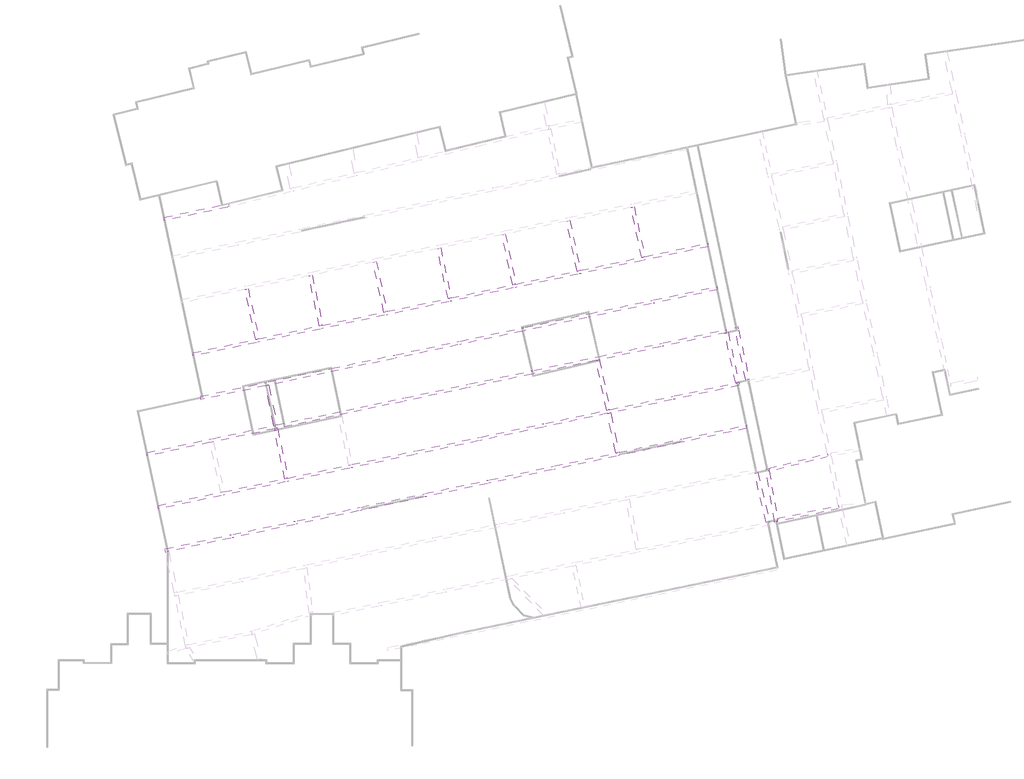
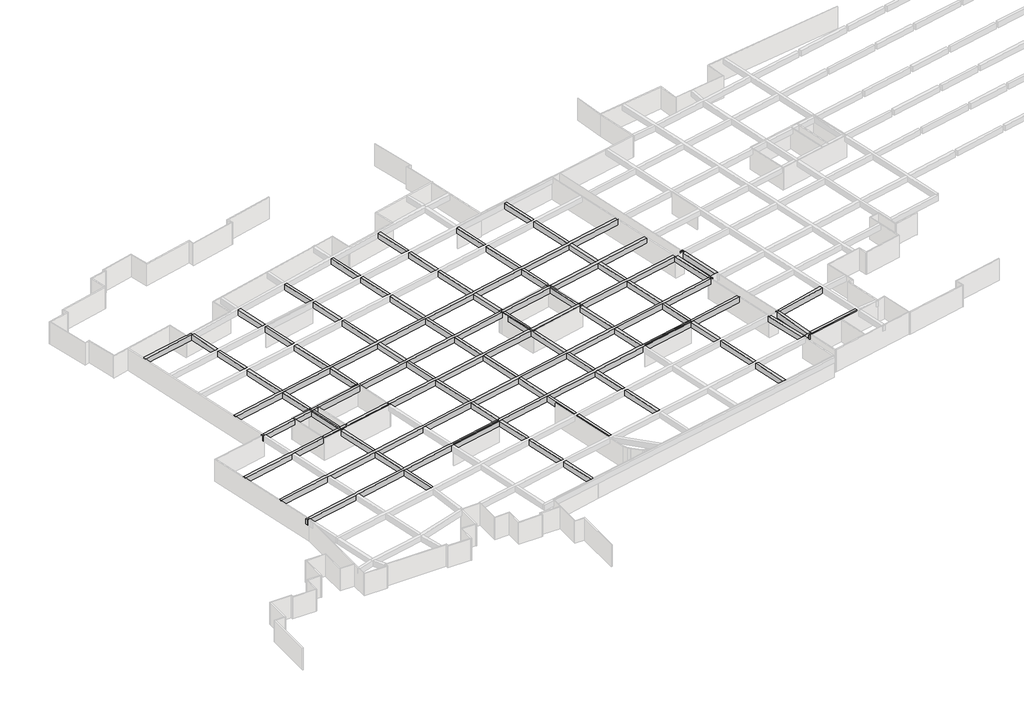
# One storey, part 8 of 14: 23 beams.
"""IFC4 building model written with IfcOpenShell, lengths in millimetres."""

from ifc_helpers import new_model, si_unit, frame, origin, place, context, project, spatial, polyline, outline, extrude, faceted_brep, element, save

model = new_model("IFC4")

# Units and contexts
model_context = context("Model", 3, world=origin())
ifc_project = project(units=[si_unit("LENGTHUNIT", "METRE", prefix="MILLI")], contexts=[model_context])

# Site, building, storey
site = spatial("IfcSite", under=ifc_project)
building = spatial("IfcBuilding", under=site)
storey = spatial("IfcBuildingStorey", under=building, Name="户型图", Elevation=0.0)

# Beams
placement = place(None, origin())
element("IfcBeam", 1, ObjectType="混凝土 - 矩形梁 : KL_beam", at=placement, inside=storey, context=model_context, shape_type="Brep", body=[
    faceted_brep([(-335089.4441213, -155154.5631684, 3300.0), (-335089.4441213, -155154.5631684, 2500.0), (-335006.2794449, -155545.8222087, 2500.0), (-335006.2794449, -155545.8222087, 3300.0), (-327178.3172304, -153881.9374755, 3300.0), (-327267.044724, -153491.8608485, 3300.0), (-327376.7281592, -153924.1110203, 3300.0), (-327178.3172304, -153881.9374755, 2500.0), (-327376.7281592, -153924.1110203, 2500.0), (-327267.044724, -153491.8608485, 2500.0)], [[[0, 1, 2, 3]], [[4, 5, 0, 3, 6]], [[7, 4, 6, 3, 2, 8]], [[9, 7, 8, 2, 1]], [[5, 9, 1, 0]], [[5, 4, 7, 9]]]),
])
element("IfcBeam", 2, ObjectType="混凝土 - 矩形梁 : KL_beam", at=placement, inside=storey, context=model_context, shape_type="Brep", body=[
    faceted_brep([(-269078.2925997, -158315.8590101, 3300.0), (-268995.1279234, -158707.1180504, 3300.0), (-268995.1279234, -158707.1180504, 2500.0), (-269078.2925997, -158315.8590101, 2500.0), (-331592.6839102, -171603.7030819, 3300.0), (-331592.6839102, -171603.7030819, 2500.0), (-331509.5192339, -171994.9621222, 2500.0), (-331509.5192339, -171994.9621222, 3300.0), (-276698.1734204, -159935.5146776, 3300.0), (-277089.4324607, -160018.679354, 3300.0), (-284525.3700507, -161599.2366809, 3300.0), (-284916.629091, -161682.4013572, 3300.0), (-292343.5420768, -163261.0404453, 3300.0), (-292734.8011171, -163344.2051217, 3300.0), (-300204.2486812, -164931.8852135, 3300.0), (-300595.5077215, -165015.0498898, 3300.0), (-308006.2318604, -166590.2479322, 3300.0), (-308397.4910792, -166673.4126465, 3300.0), (-315818.4231217, -168250.7804458, 3300.0), (-316209.682162, -168333.9451222, 3300.0), (-323572.2444184, -169898.9060405, 3300.0), (-323963.5034587, -169982.0707168, 3300.0), (-323880.3387823, -170373.3297571, 3300.0), (-323489.0797421, -170290.1650808, 3300.0), (-316126.5174857, -168725.2041625, 3300.0), (-315735.2584454, -168642.0394861, 3300.0), (-308313.9526955, -167064.5922528, 3300.0), (-307922.6934768, -166981.4275386, 3300.0), (-300512.3430452, -165406.3089301, 3300.0), (-300121.0840049, -165323.1442537, 3300.0), (-292651.6364408, -163735.4641619, 3300.0), (-292260.3774005, -163652.2994856, 3300.0), (-284833.4644147, -162073.6603975, 3300.0), (-284442.2053744, -161990.4957212, 3300.0), (-277006.2677843, -160409.9383943, 3300.0), (-276615.008744, -160326.7737179, 3300.0), (-323880.3387823, -170373.3297571, 2500.0), (-323489.0797421, -170290.1650808, 2500.0), (-316126.5174857, -168725.2041625, 2500.0), (-315735.2584454, -168642.0394861, 2500.0), (-308313.9526955, -167064.5922528, 2500.0), (-307922.6934768, -166981.4275386, 2500.0), (-300512.3430452, -165406.3089301, 2500.0), (-300121.0840049, -165323.1442537, 2500.0), (-292651.6364408, -163735.4641619, 2500.0), (-292260.3774005, -163652.2994856, 2500.0), (-284833.4644147, -162073.6603975, 2500.0), (-284442.2053744, -161990.4957212, 2500.0), (-277006.2677843, -160409.9383943, 2500.0), (-276615.008744, -160326.7737179, 2500.0), (-323963.5034587, -169982.0707168, 2500.0), (-323572.2444184, -169898.9060405, 2500.0), (-316209.682162, -168333.9451222, 2500.0), (-315818.4231217, -168250.7804458, 2500.0), (-308397.4910792, -166673.4126465, 2500.0), (-308006.2318604, -166590.2479322, 2500.0), (-300595.5077215, -165015.0498898, 2500.0), (-300204.2486812, -164931.8852135, 2500.0), (-292734.8011171, -163344.2051217, 2500.0), (-292343.5420768, -163261.0404453, 2500.0), (-284916.629091, -161682.4013572, 2500.0), (-284525.3700507, -161599.2366809, 2500.0), (-277089.4324607, -160018.679354, 2500.0), (-276698.1734204, -159935.5146776, 2500.0)], [[[0, 1, 2, 3]], [[4, 5, 6, 7]], [[1, 0, 8, 9, 10, 11, 12, 13, 14, 15, 16, 17, 18, 19, 20, 21, 4, 7, 22, 23, 24, 25, 26, 27, 28, 29, 30, 31, 32, 33, 34, 35]], [[2, 1, 35, 34, 33, 32, 31, 30, 29, 28, 27, 26, 25, 24, 23, 22, 7, 6, 36, 37, 38, 39, 40, 41, 42, 43, 44, 45, 46, 47, 48, 49]], [[3, 2, 49, 48, 47, 46, 45, 44, 43, 42, 41, 40, 39, 38, 37, 36, 6, 5, 50, 51, 52, 53, 54, 55, 56, 57, 58, 59, 60, 61, 62, 63]], [[0, 3, 63, 62, 61, 60, 59, 58, 57, 56, 55, 54, 53, 52, 51, 50, 5, 4, 21, 20, 19, 18, 17, 16, 15, 14, 13, 12, 11, 10, 9, 8]]]),
])
element("IfcBeam", 3, ObjectType="混凝土 - 矩形梁 : KL_beam", at=placement, inside=storey, context=model_context, shape_type="Brep", body=[
    faceted_brep([(-267962.3983208, -163565.7288339, 3300.0), (-267879.2336445, -163956.9878742, 3300.0), (-267879.2336445, -163956.9878742, 2500.0), (-267962.3983208, -163565.7288339, 2500.0), (-275582.2791414, -165185.3845014, 3300.0), (-275973.5381817, -165268.5491778, 3300.0), (-283409.4757718, -166849.1065047, 3300.0), (-283800.7348121, -166932.271181, 3300.0), (-291227.6477979, -168510.9102691, 3300.0), (-291618.9068381, -168594.0749454, 3300.0), (-299088.3544023, -170181.7550372, 3300.0), (-299479.6134426, -170264.9197136, 3300.0), (-306885.3232191, -171839.0519204, 3300.0), (-307276.5824379, -171922.2166347, 3300.0), (-314702.5288428, -173500.6502696, 3300.0), (-315093.787883, -173583.814946, 3300.0), (-322456.3501394, -175148.7758643, 3300.0), (-322847.6091797, -175231.9405406, 3300.0), (-330672.7899856, -176895.2340671, 3300.0), (-330589.6253093, -177286.4931074, 3300.0), (-330198.366269, -177203.3284311, 3300.0), (-322764.4445034, -175623.1995809, 3300.0), (-322373.1854631, -175540.0349045, 3300.0), (-307193.0440543, -172313.396241, 3300.0), (-306801.7848355, -172230.2315268, 3300.0), (-299396.4487662, -170656.1787539, 3300.0), (-299005.1897259, -170573.0140775, 3300.0), (-291535.7421618, -168985.3339857, 3300.0), (-291144.4831215, -168902.1693094, 3300.0), (-283717.5701358, -167323.5302213, 3300.0), (-283326.3110955, -167240.365545, 3300.0), (-275890.3735054, -165659.8082181, 3300.0), (-275499.1144651, -165576.6435417, 3300.0), (-330589.6253093, -177286.4931074, 2500.0), (-330198.366269, -177203.3284311, 2500.0), (-322764.4445034, -175623.1995809, 2500.0), (-322373.1854631, -175540.0349045, 2500.0), (-307193.0440543, -172313.396241, 2500.0), (-306801.7848355, -172230.2315268, 2500.0), (-299396.4487662, -170656.1787539, 2500.0), (-299005.1897259, -170573.0140775, 2500.0), (-291535.7421618, -168985.3339857, 2500.0), (-291144.4831215, -168902.1693094, 2500.0), (-283717.5701358, -167323.5302213, 2500.0), (-283326.3110955, -167240.365545, 2500.0), (-275890.3735054, -165659.8082181, 2500.0), (-275499.1144651, -165576.6435417, 2500.0), (-330672.7899856, -176895.2340671, 2500.0), (-322847.6091797, -175231.9405406, 2500.0), (-322456.3501394, -175148.7758643, 2500.0), (-315093.787883, -173583.814946, 2500.0), (-314702.5288428, -173500.6502696, 2500.0), (-307276.5824379, -171922.2166347, 2500.0), (-306885.3232191, -171839.0519204, 2500.0), (-299479.6134426, -170264.9197136, 2500.0), (-299088.3544023, -170181.7550372, 2500.0), (-291618.9068382, -168594.0749454, 2500.0), (-291227.6477979, -168510.9102691, 2500.0), (-283800.7348121, -166932.271181, 2500.0), (-283409.4757718, -166849.1065047, 2500.0), (-275973.5381817, -165268.5491778, 2500.0), (-275582.2791414, -165185.3845014, 2500.0)], [[[0, 1, 2, 3]], [[1, 0, 4, 5, 6, 7, 8, 9, 10, 11, 12, 13, 14, 15, 16, 17, 18, 19, 20, 21, 22, 23, 24, 25, 26, 27, 28, 29, 30, 31, 32]], [[2, 1, 32, 31, 30, 29, 28, 27, 26, 25, 24, 23, 22, 21, 20, 19, 33, 34, 35, 36, 37, 38, 39, 40, 41, 42, 43, 44, 45, 46]], [[3, 2, 46, 45, 44, 43, 42, 41, 40, 39, 38, 37, 36, 35, 34, 33, 47, 48, 49, 50, 51, 52, 53, 54, 55, 56, 57, 58, 59, 60, 61]], [[0, 3, 61, 60, 59, 58, 57, 56, 55, 54, 53, 52, 51, 50, 49, 48, 47, 18, 17, 16, 15, 14, 13, 12, 11, 10, 9, 8, 7, 6, 5, 4]], [[19, 18, 47, 33]]]),
])
element("IfcBeam", 4, ObjectType="混凝土 - 矩形梁 : KL_beam", at=placement, inside=storey, context=model_context, shape_type="Brep", body=[
    faceted_brep([(-266853.637508, -168782.0383379, 3300.0), (-266770.4728317, -169173.2973782, 3300.0), (-266770.4728317, -169173.2973782, 2500.0), (-266853.637508, -168782.0383379, 2500.0), (-337193.2096244, -183733.1759363, 3300.0), (-337193.2096244, -183733.1759363, 2500.0), (-337110.044948, -184124.4349766, 2500.0), (-337110.044948, -184124.4349766, 3300.0), (-274473.5183286, -170401.6940055, 3300.0), (-274864.7773689, -170484.8586818, 3300.0), (-282300.714959, -172065.4160088, 3300.0), (-282691.9739993, -172148.5806851, 3300.0), (-290118.8869851, -173727.2197732, 3300.0), (-290510.1460254, -173810.3844495, 3300.0), (-297979.5935895, -175398.0645413, 3300.0), (-298370.8526298, -175481.2292176, 3300.0), (-305771.5800988, -177054.3024023, 3300.0), (-306162.8393176, -177137.4671166, 3300.0), (-321347.5893266, -180365.0853683, 3300.0), (-321738.8483669, -180448.2500446, 3300.0), (-329172.7701325, -182028.3788949, 3300.0), (-329564.0291728, -182111.5435712, 3300.0), (-329480.8644965, -182502.8026115, 3300.0), (-329089.6054562, -182419.6379352, 3300.0), (-321655.6836906, -180839.5090849, 3300.0), (-321264.4246503, -180756.3444086, 3300.0), (-306079.3009339, -177528.6467229, 3300.0), (-305688.0417152, -177445.4820087, 3300.0), (-298287.6879534, -175872.4882579, 3300.0), (-297896.4289131, -175789.3235816, 3300.0), (-290426.981349, -174201.6434898, 3300.0), (-290035.7223087, -174118.4788135, 3300.0), (-282608.809323, -172539.8397254, 3300.0), (-282217.5502827, -172456.6750491, 3300.0), (-274781.6126926, -170876.1177221, 3300.0), (-274390.3536523, -170792.9530458, 3300.0), (-329480.8644965, -182502.8026115, 2500.0), (-329089.6054562, -182419.6379352, 2500.0), (-321655.6836906, -180839.5090849, 2500.0), (-321264.4246503, -180756.3444086, 2500.0), (-306079.3009339, -177528.6467229, 2500.0), (-305688.0417152, -177445.4820087, 2500.0), (-298287.6879534, -175872.4882579, 2500.0), (-297896.4289131, -175789.3235816, 2500.0), (-290426.981349, -174201.6434898, 2500.0), (-290035.7223087, -174118.4788135, 2500.0), (-282608.809323, -172539.8397254, 2500.0), (-282217.5502827, -172456.6750491, 2500.0), (-274781.6126926, -170876.1177221, 2500.0), (-274390.3536523, -170792.9530458, 2500.0), (-329564.0291728, -182111.5435712, 2500.0), (-329172.7701325, -182028.3788949, 2500.0), (-321738.8483669, -180448.2500446, 2500.0), (-321347.5893266, -180365.0853683, 2500.0), (-306162.8393176, -177137.4671166, 2500.0), (-305771.5800988, -177054.3024023, 2500.0), (-298370.8526298, -175481.2292176, 2500.0), (-297979.5935895, -175398.0645413, 2500.0), (-290510.1460254, -173810.3844495, 2500.0), (-290118.8869851, -173727.2197732, 2500.0), (-282691.9739993, -172148.5806851, 2500.0), (-282300.714959, -172065.4160088, 2500.0), (-274864.7773689, -170484.8586818, 2500.0), (-274473.5183286, -170401.6940055, 2500.0)], [[[0, 1, 2, 3]], [[4, 5, 6, 7]], [[1, 0, 8, 9, 10, 11, 12, 13, 14, 15, 16, 17, 18, 19, 20, 21, 4, 7, 22, 23, 24, 25, 26, 27, 28, 29, 30, 31, 32, 33, 34, 35]], [[2, 1, 35, 34, 33, 32, 31, 30, 29, 28, 27, 26, 25, 24, 23, 22, 7, 6, 36, 37, 38, 39, 40, 41, 42, 43, 44, 45, 46, 47, 48, 49]], [[3, 2, 49, 48, 47, 46, 45, 44, 43, 42, 41, 40, 39, 38, 37, 36, 6, 5, 50, 51, 52, 53, 54, 55, 56, 57, 58, 59, 60, 61, 62, 63]], [[0, 3, 63, 62, 61, 60, 59, 58, 57, 56, 55, 54, 53, 52, 51, 50, 5, 4, 21, 20, 19, 18, 17, 16, 15, 14, 13, 12, 11, 10, 9, 8]]]),
])
element("IfcBeam", 5, ObjectType="混凝土 - 矩形梁 : KL_beam", at=placement, inside=storey, context=model_context, shape_type="Brep", body=[
    faceted_brep([(-335824.1162075, -190174.2540481, 3300.0), (-335824.1162075, -190174.2540481, 2500.0), (-335740.9515311, -190565.5130884, 2500.0), (-335740.9515311, -190565.5130884, 3300.0), (-328111.7710796, -188943.8807233, 3300.0), (-327720.5120393, -188860.7160469, 3300.0), (-320340.639733, -187292.0757639, 3300.0), (-319949.3806927, -187208.9110876, 3300.0), (-312559.6270999, -185638.1704723, 3300.0), (-312168.3680596, -185555.005796, 3300.0), (-304704.0553837, -183968.4171584, 3300.0), (-304312.7961649, -183885.2524441, 3300.0), (-296918.5945366, -182313.5663697, 3300.0), (-296527.3354963, -182230.4016934, 3300.0), (-289057.8879321, -180642.7216016, 3300.0), (-288666.6288918, -180559.5569253, 3300.0), (-281239.7159061, -178980.9178372, 3300.0), (-280848.4568658, -178897.7531609, 3300.0), (-273412.5192757, -177317.1958339, 3300.0), (-273021.2602354, -177234.0311576, 3300.0), (-265205.3790605, -175572.7143286, 3300.0), (-265288.5437368, -175181.4552883, 3300.0), (-265679.8027771, -175264.6199647, 3300.0), (-273104.4249117, -176842.7721173, 3300.0), (-273495.683952, -176925.9367936, 3300.0), (-280931.6215421, -178506.4941206, 3300.0), (-281322.8805824, -178589.6587969, 3300.0), (-288749.7935682, -180168.297885, 3300.0), (-289141.0526085, -180251.4625613, 3300.0), (-296610.5001726, -181839.1426531, 3300.0), (-297001.7592129, -181922.3073294, 3300.0), (-304396.3345485, -183494.0728378, 3300.0), (-304787.5937673, -183577.237552, 3300.0), (-312251.5327359, -185163.7467557, 3300.0), (-312642.7917762, -185246.9114321, 3300.0), (-320032.545369, -186817.6520473, 3300.0), (-320423.8044093, -186900.8167236, 3300.0), (-327803.6767156, -188469.4570066, 3300.0), (-328194.9357559, -188552.621683, 3300.0), (-328111.7710796, -188943.8807233, 2500.0), (-327720.5120393, -188860.7160469, 2500.0), (-320340.639733, -187292.0757639, 2500.0), (-319949.3806927, -187208.9110876, 2500.0), (-312559.6270999, -185638.1704723, 2500.0), (-312168.3680596, -185555.005796, 2500.0), (-304704.0553837, -183968.4171584, 2500.0), (-304312.7961649, -183885.2524441, 2500.0), (-296918.5945366, -182313.5663697, 2500.0), (-296527.3354963, -182230.4016934, 2500.0), (-289057.8879321, -180642.7216016, 2500.0), (-288666.6288918, -180559.5569253, 2500.0), (-281239.7159061, -178980.9178372, 2500.0), (-280848.4568658, -178897.7531609, 2500.0), (-273412.5192757, -177317.1958339, 2500.0), (-273021.2602354, -177234.0311576, 2500.0), (-265205.3790605, -175572.7143286, 2500.0), (-328194.9357559, -188552.621683, 2500.0), (-327803.6767156, -188469.4570066, 2500.0), (-320423.8044093, -186900.8167236, 2500.0), (-320032.545369, -186817.6520473, 2500.0), (-312642.7917762, -185246.9114321, 2500.0), (-312251.5327359, -185163.7467557, 2500.0), (-304787.5937673, -183577.237552, 2500.0), (-304396.3345485, -183494.0728378, 2500.0), (-297001.7592129, -181922.3073294, 2500.0), (-296610.5001726, -181839.1426531, 2500.0), (-289141.0526085, -180251.4625613, 2500.0), (-288749.7935682, -180168.297885, 2500.0), (-281322.8805824, -178589.6587969, 2500.0), (-280931.6215421, -178506.4941206, 2500.0), (-273495.683952, -176925.9367936, 2500.0), (-273104.4249117, -176842.7721173, 2500.0), (-265679.8027771, -175264.6199647, 2500.0), (-265288.5437368, -175181.4552883, 2500.0)], [[[0, 1, 2, 3]], [[0, 3, 4, 5, 6, 7, 8, 9, 10, 11, 12, 13, 14, 15, 16, 17, 18, 19, 20, 21, 22, 23, 24, 25, 26, 27, 28, 29, 30, 31, 32, 33, 34, 35, 36, 37, 38]], [[3, 2, 39, 40, 41, 42, 43, 44, 45, 46, 47, 48, 49, 50, 51, 52, 53, 54, 55, 20, 19, 18, 17, 16, 15, 14, 13, 12, 11, 10, 9, 8, 7, 6, 5, 4]], [[2, 1, 56, 57, 58, 59, 60, 61, 62, 63, 64, 65, 66, 67, 68, 69, 70, 71, 72, 73, 55, 54, 53, 52, 51, 50, 49, 48, 47, 46, 45, 44, 43, 42, 41, 40, 39]], [[1, 0, 38, 37, 36, 35, 34, 33, 32, 31, 30, 29, 28, 27, 26, 25, 24, 23, 22, 21, 73, 72, 71, 70, 69, 68, 67, 66, 65, 64, 63, 62, 61, 60, 59, 58, 57, 56]], [[21, 20, 55, 73]]]),
])
element("IfcBeam", 6, ObjectType="混凝土 - 矩形梁 : KL_beam", at=placement, inside=storey, context=model_context, shape_type="Brep", body=[
    faceted_brep([(-264398.9072597, -180410.7623704, 3300.0), (-264315.7425834, -180802.0214107, 3300.0), (-264315.7425834, -180802.0214107, 2500.0), (-264398.9072597, -180410.7623704, 2500.0), (-272002.4929504, -182026.9544012, 3300.0), (-272393.7519907, -182110.1190775, 3300.0), (-279829.6895808, -183690.6764045, 3300.0), (-280220.9486211, -183773.8410808, 3300.0), (-287647.8616068, -185352.4801689, 3300.0), (-288039.1206471, -185435.6448452, 3300.0), (-295508.5682113, -187023.324937, 3300.0), (-295899.8272515, -187106.4896133, 3300.0), (-303289.4509656, -188677.202622, 3300.0), (-303680.7101844, -188760.3673363, 3300.0), (-311149.6007746, -190347.9290396, 3300.0), (-311540.8598149, -190431.0937159, 3300.0), (-318930.6134077, -192001.8343312, 3300.0), (-319321.8724479, -192084.9990075, 3300.0), (-326701.7447543, -193653.6392905, 3300.0), (-327093.0037946, -193736.8039669, 3300.0), (-334976.648082, -195412.52429, 3300.0), (-334893.4834057, -195803.7833303, 3300.0), (-334502.2243654, -195720.618654, 3300.0), (-327009.8391182, -194128.0630072, 3300.0), (-326618.580078, -194044.8983308, 3300.0), (-319238.7077716, -192476.2580478, 3300.0), (-318847.4487313, -192393.0933715, 3300.0), (-311457.6951385, -190822.3527562, 3300.0), (-311066.4360982, -190739.1880799, 3300.0), (-303597.1718008, -189151.5469426, 3300.0), (-303205.912582, -189068.3822284, 3300.0), (-295816.6625752, -187497.7486536, 3300.0), (-295425.4035349, -187414.5839773, 3300.0), (-287955.9559708, -185826.9038855, 3300.0), (-287564.6969305, -185743.7392092, 3300.0), (-280137.7839447, -184165.1001211, 3300.0), (-279746.5249044, -184081.9354447, 3300.0), (-272310.5873144, -182501.3781178, 3300.0), (-271919.3282741, -182418.2134415, 3300.0), (-334893.4834057, -195803.7833303, 2500.0), (-334502.2243654, -195720.618654, 2500.0), (-327009.8391182, -194128.0630072, 2500.0), (-326618.580078, -194044.8983308, 2500.0), (-319238.7077716, -192476.2580478, 2500.0), (-318847.4487313, -192393.0933715, 2500.0), (-311457.6951385, -190822.3527562, 2500.0), (-311066.4360982, -190739.1880799, 2500.0), (-303597.1718008, -189151.5469426, 2500.0), (-303205.912582, -189068.3822284, 2500.0), (-295816.6625752, -187497.7486536, 2500.0), (-295425.4035349, -187414.5839773, 2500.0), (-287955.9559708, -185826.9038855, 2500.0), (-287564.6969305, -185743.7392092, 2500.0), (-280137.7839447, -184165.1001211, 2500.0), (-279746.5249044, -184081.9354447, 2500.0), (-272310.5873144, -182501.3781178, 2500.0), (-271919.3282741, -182418.2134415, 2500.0), (-334976.648082, -195412.52429, 2500.0), (-327093.0037946, -193736.8039669, 2500.0), (-326701.7447543, -193653.6392905, 2500.0), (-319321.8724479, -192084.9990075, 2500.0), (-318930.6134077, -192001.8343312, 2500.0), (-311540.8598149, -190431.0937159, 2500.0), (-311149.6007746, -190347.9290396, 2500.0), (-303680.7101844, -188760.3673363, 2500.0), (-303289.4509656, -188677.202622, 2500.0), (-295899.8272515, -187106.4896133, 2500.0), (-295508.5682113, -187023.324937, 2500.0), (-288039.1206471, -185435.6448452, 2500.0), (-287647.8616068, -185352.4801689, 2500.0), (-280220.9486211, -183773.8410808, 2500.0), (-279829.6895808, -183690.6764045, 2500.0), (-272393.7519907, -182110.1190775, 2500.0), (-272002.4929504, -182026.9544012, 2500.0)], [[[0, 1, 2, 3]], [[1, 0, 4, 5, 6, 7, 8, 9, 10, 11, 12, 13, 14, 15, 16, 17, 18, 19, 20, 21, 22, 23, 24, 25, 26, 27, 28, 29, 30, 31, 32, 33, 34, 35, 36, 37, 38]], [[2, 1, 38, 37, 36, 35, 34, 33, 32, 31, 30, 29, 28, 27, 26, 25, 24, 23, 22, 21, 39, 40, 41, 42, 43, 44, 45, 46, 47, 48, 49, 50, 51, 52, 53, 54, 55, 56]], [[3, 2, 56, 55, 54, 53, 52, 51, 50, 49, 48, 47, 46, 45, 44, 43, 42, 41, 40, 39, 57, 58, 59, 60, 61, 62, 63, 64, 65, 66, 67, 68, 69, 70, 71, 72, 73]], [[0, 3, 73, 72, 71, 70, 69, 68, 67, 66, 65, 64, 63, 62, 61, 60, 59, 58, 57, 20, 19, 18, 17, 16, 15, 14, 13, 12, 11, 10, 9, 8, 7, 6, 5, 4]], [[21, 20, 57, 39]]]),
])
element("IfcBeam", 7, ObjectType="混凝土 - 矩形梁 : KL_beam", at=placement, inside=storey, context=model_context, shape_type="SweptSolid", body=[
    extrude(outline(polyline([(-322456.3501394, -175148.7758643), (-322847.6091797, -175231.9405406), (-323880.3387823, -170373.3297571), (-323489.0797421, -170290.1650808), (-322456.3501394, -175148.7758643)])), frame((0.0, 0.0, 2500.0), z_axis=(0.0, 0.0, 1.0), x_axis=(1.0, 0.0, 0.0)), (0.0, 0.0, 1.0), 800.0),
    extrude(outline(polyline([(-327376.7281592, -153924.1110203), (-327178.3172304, -153881.9374755), (-326986.6349567, -153835.4615086), (-326070.6576793, -158144.7957872), (-326461.9167196, -158227.9604635), (-327376.7281592, -153924.1110203)])), frame((0.0, 0.0, 2500.0), z_axis=(0.0, 0.0, 1.0), x_axis=(1.0, 0.0, 0.0)), (0.0, 0.0, 1.0), 800.0),
    extrude(outline(polyline([(-326378.7520433, -158619.2195038), (-325987.493003, -158536.0548275), (-324943.7763151, -163446.3557832), (-325335.0353554, -163529.5204595), (-326378.7520433, -158619.2195038)])), frame((0.0, 0.0, 2500.0), z_axis=(0.0, 0.0, 1.0), x_axis=(1.0, 0.0, 0.0)), (0.0, 0.0, 1.0), 800.0),
    extrude(outline(polyline([(-325251.870679, -163920.7794998), (-324860.6116388, -163837.6148234), (-323572.2444184, -169898.9060405), (-323963.5034587, -169982.0707168), (-325251.870679, -163920.7794998)])), frame((0.0, 0.0, 2500.0), z_axis=(0.0, 0.0, 1.0), x_axis=(1.0, 0.0, 0.0)), (0.0, 0.0, 1.0), 800.0),
])
element("IfcBeam", 8, ObjectType="混凝土 - 矩形梁 : KL_beam", at=placement, inside=storey, context=model_context, shape_type="SweptSolid", body=[
    extrude(outline(polyline([(-314702.5288428, -173500.6502696), (-315093.787883, -173583.814946), (-316126.5174857, -168725.2041625), (-315735.2584454, -168642.0394861), (-314702.5288428, -173500.6502696)])), frame((0.0, 0.0, 2500.0), z_axis=(0.0, 0.0, 1.0), x_axis=(1.0, 0.0, 0.0)), (0.0, 0.0, 1.0), 800.0),
    extrude(outline(polyline([(-319668.5820962, -152061.1003462), (-319279.6883606, -151966.8077859), (-318316.8363826, -156496.6701926), (-318708.0954229, -156579.8348689), (-319668.5820962, -152061.1003462)])), frame((0.0, 0.0, 2500.0), z_axis=(0.0, 0.0, 1.0), x_axis=(1.0, 0.0, 0.0)), (0.0, 0.0, 1.0), 800.0),
    extrude(outline(polyline([(-318624.9307466, -156971.0939092), (-318233.6717063, -156887.9292328), (-317189.9550184, -161798.2301885), (-317581.2140587, -161881.3948649), (-318624.9307466, -156971.0939092)])), frame((0.0, 0.0, 2500.0), z_axis=(0.0, 0.0, 1.0), x_axis=(1.0, 0.0, 0.0)), (0.0, 0.0, 1.0), 800.0),
    extrude(outline(polyline([(-317498.0493824, -162272.6539051), (-317106.7903421, -162189.4892288), (-315818.4231217, -168250.7804458), (-316209.682162, -168333.9451222), (-317498.0493824, -162272.6539051)])), frame((0.0, 0.0, 2500.0), z_axis=(0.0, 0.0, 1.0), x_axis=(1.0, 0.0, 0.0)), (0.0, 0.0, 1.0), 800.0),
])
element("IfcBeam", 9, ObjectType="混凝土 - 矩形梁 : KL_beam", at=placement, inside=storey, context=model_context, shape_type="SweptSolid", body=[
    extrude(outline(polyline([(-299656.3845067, -205689.5201441), (-300048.0525146, -205770.7706487), (-301119.8402372, -200751.981904), (-300728.1722293, -200670.7313994), (-299656.3845067, -205689.5201441)])), frame((0.0, 0.0, 2500.0), z_axis=(0.0, 0.0, 1.0), x_axis=(1.0, 0.0, 0.0)), (0.0, 0.0, 1.0), 800.0),
    extrude(outline(polyline([(-311919.2779813, -150182.1764686), (-311530.3946325, -150087.8864267), (-310515.8719459, -154838.5240142), (-310907.1311647, -154921.6887284), (-311919.2779813, -150182.1764686)])), frame((0.0, 0.0, 2500.0), z_axis=(0.0, 0.0, 1.0), x_axis=(1.0, 0.0, 0.0)), (0.0, 0.0, 1.0), 800.0),
    extrude(outline(polyline([(-310823.5927811, -155312.8683348), (-310432.3335623, -155229.7036205), (-309383.926848, -160139.0076803), (-309775.1860668, -160222.1723946), (-310823.5927811, -155312.8683348)])), frame((0.0, 0.0, 2500.0), z_axis=(0.0, 0.0, 1.0), x_axis=(1.0, 0.0, 0.0)), (0.0, 0.0, 1.0), 800.0),
    extrude(outline(polyline([(-309691.6476832, -160613.3520009), (-309300.3884644, -160530.1872867), (-308006.2318604, -166590.2479322), (-308397.4910792, -166673.4126465), (-309691.6476832, -160613.3520009)])), frame((0.0, 0.0, 2500.0), z_axis=(0.0, 0.0, 1.0), x_axis=(1.0, 0.0, 0.0)), (0.0, 0.0, 1.0), 800.0),
    extrude(outline(polyline([(-308313.9526955, -167064.5922528), (-307922.6934768, -166981.4275386), (-306885.3232191, -171839.0519204), (-307276.5824379, -171922.2166347), (-308313.9526955, -167064.5922528)])), frame((0.0, 0.0, 2500.0), z_axis=(0.0, 0.0, 1.0), x_axis=(1.0, 0.0, 0.0)), (0.0, 0.0, 1.0), 800.0),
    extrude(outline(polyline([(-307193.0440543, -172313.396241), (-306801.7848355, -172230.2315268), (-305771.5800988, -177054.3024023), (-306162.8393176, -177137.4671166), (-307193.0440543, -172313.396241)])), frame((0.0, 0.0, 2500.0), z_axis=(0.0, 0.0, 1.0), x_axis=(1.0, 0.0, 0.0)), (0.0, 0.0, 1.0), 800.0),
    extrude(outline(polyline([(-306079.3009339, -177528.6467229), (-305688.0417152, -177445.4820087), (-304396.3345485, -183494.0728378), (-304787.5937673, -183577.237552), (-306079.3009339, -177528.6467229)])), frame((0.0, 0.0, 2500.0), z_axis=(0.0, 0.0, 1.0), x_axis=(1.0, 0.0, 0.0)), (0.0, 0.0, 1.0), 800.0),
    extrude(outline(polyline([(-304704.0553837, -183968.4171584), (-304312.7961649, -183885.2524441), (-303289.4509656, -188677.202622), (-303680.7101844, -188760.3673363), (-304704.0553837, -183968.4171584)])), frame((0.0, 0.0, 2500.0), z_axis=(0.0, 0.0, 1.0), x_axis=(1.0, 0.0, 0.0)), (0.0, 0.0, 1.0), 800.0),
    extrude(outline(polyline([(-303597.1718008, -189151.5469426), (-303205.912582, -189068.3822284), (-302149.0676913, -194017.1991728), (-302540.3269101, -194100.3638871), (-303597.1718008, -189151.5469426)])), frame((0.0, 0.0, 2500.0), z_axis=(0.0, 0.0, 1.0), x_axis=(1.0, 0.0, 0.0)), (0.0, 0.0, 1.0), 800.0),
    extrude(outline(polyline([(-302456.7885265, -194491.5434934), (-302065.5293077, -194408.3787792), (-300811.7120035, -200279.5452813), (-301203.3800115, -200360.7957858), (-302456.7885265, -194491.5434934)])), frame((0.0, 0.0, 2500.0), z_axis=(0.0, 0.0, 1.0), x_axis=(1.0, 0.0, 0.0)), (0.0, 0.0, 1.0), 800.0),
])
element("IfcBeam", 10, ObjectType="混凝土 - 矩形梁 : KL_beam", at=placement, inside=storey, context=model_context, shape_type="SweptSolid", body=[
    extrude(outline(polyline([(-293033.8318018, -198666.0443617), (-293425.4978005, -198747.2944494), (-294681.3807826, -192838.8295578), (-294290.1217423, -192755.6648815), (-293033.8318018, -198666.0443617)])), frame((0.0, 0.0, 2500.0), z_axis=(0.0, 0.0, 1.0), x_axis=(1.0, 0.0, 0.0)), (0.0, 0.0, 1.0), 800.0),
    extrude(outline(polyline([(-304148.8010812, -148298.1189621), (-303759.9073457, -148203.8264018), (-302702.6619422, -153177.7749602), (-303093.9209824, -153260.9396365), (-304148.8010812, -148298.1189621)])), frame((0.0, 0.0, 2500.0), z_axis=(0.0, 0.0, 1.0), x_axis=(1.0, 0.0, 0.0)), (0.0, 0.0, 1.0), 800.0),
    extrude(outline(polyline([(-303010.7563061, -153652.1986768), (-302619.4972658, -153569.0340005), (-301575.7805779, -158479.3349561), (-301967.0396182, -158562.4996325), (-303010.7563061, -153652.1986768)])), frame((0.0, 0.0, 2500.0), z_axis=(0.0, 0.0, 1.0), x_axis=(1.0, 0.0, 0.0)), (0.0, 0.0, 1.0), 800.0),
    extrude(outline(polyline([(-301883.8749419, -158953.7586728), (-301492.6159016, -158870.5939964), (-300204.2486812, -164931.8852135), (-300595.5077215, -165015.0498898), (-301883.8749419, -158953.7586728)])), frame((0.0, 0.0, 2500.0), z_axis=(0.0, 0.0, 1.0), x_axis=(1.0, 0.0, 0.0)), (0.0, 0.0, 1.0), 800.0),
    extrude(outline(polyline([(-300512.3430452, -165406.3089301), (-300121.0840049, -165323.1442537), (-299088.3544023, -170181.7550372), (-299479.6134426, -170264.9197136), (-300512.3430452, -165406.3089301)])), frame((0.0, 0.0, 2500.0), z_axis=(0.0, 0.0, 1.0), x_axis=(1.0, 0.0, 0.0)), (0.0, 0.0, 1.0), 800.0),
    extrude(outline(polyline([(-299396.4487662, -170656.1787539), (-299005.1897259, -170573.0140775), (-297979.5935895, -175398.0645413), (-298370.8526298, -175481.2292176), (-299396.4487662, -170656.1787539)])), frame((0.0, 0.0, 2500.0), z_axis=(0.0, 0.0, 1.0), x_axis=(1.0, 0.0, 0.0)), (0.0, 0.0, 1.0), 800.0),
    extrude(outline(polyline([(-298287.6879534, -175872.4882579), (-297896.4289131, -175789.3235816), (-296610.5001726, -181839.1426531), (-297001.7592129, -181922.3073294), (-298287.6879534, -175872.4882579)])), frame((0.0, 0.0, 2500.0), z_axis=(0.0, 0.0, 1.0), x_axis=(1.0, 0.0, 0.0)), (0.0, 0.0, 1.0), 800.0),
    extrude(outline(polyline([(-296918.5945366, -182313.5663697), (-296527.3354963, -182230.4016934), (-295508.5682113, -187023.324937), (-295899.8272515, -187106.4896133), (-296918.5945366, -182313.5663697)])), frame((0.0, 0.0, 2500.0), z_axis=(0.0, 0.0, 1.0), x_axis=(1.0, 0.0, 0.0)), (0.0, 0.0, 1.0), 800.0),
    extrude(outline(polyline([(-295816.6625752, -187497.7486536), (-295425.4035349, -187414.5839773), (-294373.2864186, -192364.4058412), (-294764.5454589, -192447.5705175), (-295816.6625752, -187497.7486536)])), frame((0.0, 0.0, 2500.0), z_axis=(0.0, 0.0, 1.0), x_axis=(1.0, 0.0, 0.0)), (0.0, 0.0, 1.0), 800.0),
])
element("IfcBeam", 11, ObjectType="混凝土 - 矩形梁 : KL_beam", at=placement, inside=storey, context=model_context, shape_type="SweptSolid", body=[
    extrude(outline(polyline([(-296335.6153384, -146403.7061174), (-295946.7216029, -146309.4135571), (-294841.9553377, -151506.930192), (-295233.214378, -151590.0948684), (-296335.6153384, -146403.7061174)])), frame((0.0, 0.0, 2500.0), z_axis=(0.0, 0.0, 1.0), x_axis=(1.0, 0.0, 0.0)), (0.0, 0.0, 1.0), 800.0),
    extrude(outline(polyline([(-285164.9490789, -197033.6652069), (-285556.6150776, -197114.9152947), (-286820.6741782, -191167.9847897), (-286429.4151379, -191084.8201134), (-285164.9490789, -197033.6652069)])), frame((0.0, 0.0, 2500.0), z_axis=(0.0, 0.0, 1.0), x_axis=(1.0, 0.0, 0.0)), (0.0, 0.0, 1.0), 800.0),
    extrude(outline(polyline([(-295150.0497017, -151981.3539087), (-294758.7906614, -151898.1892323), (-293715.0739735, -156808.490188), (-294106.3330138, -156891.6548643), (-295150.0497017, -151981.3539087)])), frame((0.0, 0.0, 2500.0), z_axis=(0.0, 0.0, 1.0), x_axis=(1.0, 0.0, 0.0)), (0.0, 0.0, 1.0), 800.0),
    extrude(outline(polyline([(-294023.1683375, -157282.9139046), (-293631.9092972, -157199.7492283), (-292343.5420768, -163261.0404453), (-292734.8011171, -163344.2051217), (-294023.1683375, -157282.9139046)])), frame((0.0, 0.0, 2500.0), z_axis=(0.0, 0.0, 1.0), x_axis=(1.0, 0.0, 0.0)), (0.0, 0.0, 1.0), 800.0),
    extrude(outline(polyline([(-292651.6364408, -163735.4641619), (-292260.3774005, -163652.2994856), (-291227.6477979, -168510.9102691), (-291618.9068381, -168594.0749454), (-292651.6364408, -163735.4641619)])), frame((0.0, 0.0, 2500.0), z_axis=(0.0, 0.0, 1.0), x_axis=(1.0, 0.0, 0.0)), (0.0, 0.0, 1.0), 800.0),
    extrude(outline(polyline([(-291535.7421618, -168985.3339857), (-291144.4831215, -168902.1693094), (-290118.8869851, -173727.2197732), (-290510.1460254, -173810.3844495), (-291535.7421618, -168985.3339857)])), frame((0.0, 0.0, 2500.0), z_axis=(0.0, 0.0, 1.0), x_axis=(1.0, 0.0, 0.0)), (0.0, 0.0, 1.0), 800.0),
    extrude(outline(polyline([(-290426.981349, -174201.6434898), (-290035.7223087, -174118.4788135), (-288749.7935682, -180168.297885), (-289141.0526085, -180251.4625613), (-290426.981349, -174201.6434898)])), frame((0.0, 0.0, 2500.0), z_axis=(0.0, 0.0, 1.0), x_axis=(1.0, 0.0, 0.0)), (0.0, 0.0, 1.0), 800.0),
    extrude(outline(polyline([(-289057.8879321, -180642.7216016), (-288666.6288918, -180559.5569253), (-287647.8616068, -185352.4801689), (-288039.1206471, -185435.6448452), (-289057.8879321, -180642.7216016)])), frame((0.0, 0.0, 2500.0), z_axis=(0.0, 0.0, 1.0), x_axis=(1.0, 0.0, 0.0)), (0.0, 0.0, 1.0), 800.0),
    extrude(outline(polyline([(-287955.9559708, -185826.9038855), (-287564.6969305, -185743.7392092), (-286512.5798142, -190693.5610731), (-286903.8388545, -190776.7257494), (-287955.9559708, -185826.9038855)])), frame((0.0, 0.0, 2500.0), z_axis=(0.0, 0.0, 1.0), x_axis=(1.0, 0.0, 0.0)), (0.0, 0.0, 1.0), 800.0),
])
element("IfcBeam", 12, ObjectType="混凝土 - 矩形梁 : KL_beam", at=placement, inside=storey, context=model_context, shape_type="SweptSolid", body=[
    extrude(outline(polyline([(-281239.7159061, -178980.9178372), (-280848.4568658, -178897.7531609), (-279829.6895808, -183690.6764045), (-280220.9486211, -183773.8410808), (-281239.7159061, -178980.9178372)])), frame((0.0, 0.0, 2500.0), z_axis=(0.0, 0.0, 1.0), x_axis=(1.0, 0.0, 0.0)), (0.0, 0.0, 1.0), 800.0),
])
element("IfcBeam", 13, ObjectType="混凝土 - 矩形梁 : KL_beam", at=placement, inside=storey, context=model_context, shape_type="SweptSolid", body=[
    extrude(outline(polyline([(-282608.809323, -172539.8397254), (-282217.5502827, -172456.6750491), (-280931.6215421, -178506.4941206), (-281322.8805824, -178589.6587969), (-282608.809323, -172539.8397254)])), frame((0.0, 0.0, 2500.0), z_axis=(0.0, 0.0, 1.0), x_axis=(1.0, 0.0, 0.0)), (0.0, 0.0, 1.0), 800.0),
])
element("IfcBeam", 14, ObjectType="混凝土 - 矩形梁 : KL_beam", at=placement, inside=storey, context=model_context, shape_type="SweptSolid", body=[
    extrude(outline(polyline([(-282300.714959, -172065.4160088), (-282691.9739993, -172148.5806851), (-283717.5701358, -167323.5302213), (-283326.3110955, -167240.365545), (-282300.714959, -172065.4160088)])), frame((0.0, 0.0, 2500.0), z_axis=(0.0, 0.0, 1.0), x_axis=(1.0, 0.0, 0.0)), (0.0, 0.0, 1.0), 800.0),
    extrude(outline(polyline([(-287331.8776756, -150319.5501442), (-286940.6186353, -150236.3854679), (-285896.9019474, -155146.6864236), (-286288.1609877, -155229.8510999), (-287331.8776756, -150319.5501442)])), frame((0.0, 0.0, 2500.0), z_axis=(0.0, 0.0, 1.0), x_axis=(1.0, 0.0, 0.0)), (0.0, 0.0, 1.0), 800.0),
    extrude(outline(polyline([(-286204.9963114, -155621.1101402), (-285813.7372711, -155537.9454639), (-284525.3700507, -161599.2366809), (-284916.629091, -161682.4013572), (-286204.9963114, -155621.1101402)])), frame((0.0, 0.0, 2500.0), z_axis=(0.0, 0.0, 1.0), x_axis=(1.0, 0.0, 0.0)), (0.0, 0.0, 1.0), 800.0),
    extrude(outline(polyline([(-284833.4644147, -162073.6603975), (-284442.2053744, -161990.4957212), (-283409.4757718, -166849.1065047), (-283800.7348121, -166932.271181), (-284833.4644147, -162073.6603975)])), frame((0.0, 0.0, 2500.0), z_axis=(0.0, 0.0, 1.0), x_axis=(1.0, 0.0, 0.0)), (0.0, 0.0, 1.0), 800.0),
])
element("IfcBeam", 15, ObjectType="混凝土 - 矩形梁 : KL_beam", at=placement, inside=storey, context=model_context, shape_type="SweptSolid", body=[
    extrude(outline(polyline([(-268353.1534946, -199195.7466848), (-268744.8194932, -199276.9967726), (-269811.8076079, -194257.2123617), (-269420.1416092, -194175.962274), (-268353.1534946, -199195.7466848)])), frame((0.0, 0.0, 2500.0), z_axis=(0.0, 0.0, 1.0), x_axis=(1.0, 0.0, 0.0)), (0.0, 0.0, 1.0), 800.0),
    extrude(outline(polyline([(-279504.6810453, -148655.828141), (-279113.422005, -148572.6634647), (-278069.7053171, -153482.9644203), (-278460.9643574, -153566.1290967), (-279504.6810453, -148655.828141)])), frame((0.0, 0.0, 2500.0), z_axis=(0.0, 0.0, 1.0), x_axis=(1.0, 0.0, 0.0)), (0.0, 0.0, 1.0), 800.0),
    extrude(outline(polyline([(-278377.799681, -153957.388137), (-277986.5406407, -153874.2234606), (-276698.1734204, -159935.5146776), (-277089.4324607, -160018.679354), (-278377.799681, -153957.388137)])), frame((0.0, 0.0, 2500.0), z_axis=(0.0, 0.0, 1.0), x_axis=(1.0, 0.0, 0.0)), (0.0, 0.0, 1.0), 800.0),
    extrude(outline(polyline([(-277006.2677843, -160409.9383943), (-276615.008744, -160326.7737179), (-275582.2791414, -165185.3845014), (-275973.5381817, -165268.5491778), (-277006.2677843, -160409.9383943)])), frame((0.0, 0.0, 2500.0), z_axis=(0.0, 0.0, 1.0), x_axis=(1.0, 0.0, 0.0)), (0.0, 0.0, 1.0), 800.0),
    extrude(outline(polyline([(-275890.3735054, -165659.8082181), (-275499.1144651, -165576.6435417), (-274473.5183286, -170401.6940055), (-274864.7773689, -170484.8586818), (-275890.3735054, -165659.8082181)])), frame((0.0, 0.0, 2500.0), z_axis=(0.0, 0.0, 1.0), x_axis=(1.0, 0.0, 0.0)), (0.0, 0.0, 1.0), 800.0),
    extrude(outline(polyline([(-274781.6126926, -170876.1177221), (-274390.3536523, -170792.9530458), (-273104.4249117, -176842.7721173), (-273495.683952, -176925.9367936), (-274781.6126926, -170876.1177221)])), frame((0.0, 0.0, 2500.0), z_axis=(0.0, 0.0, 1.0), x_axis=(1.0, 0.0, 0.0)), (0.0, 0.0, 1.0), 800.0),
    extrude(outline(polyline([(-273412.5192757, -177317.1958339), (-273021.2602354, -177234.0311576), (-272002.4929504, -182026.9544012), (-272393.7519907, -182110.1190775), (-273412.5192757, -177317.1958339)])), frame((0.0, 0.0, 2500.0), z_axis=(0.0, 0.0, 1.0), x_axis=(1.0, 0.0, 0.0)), (0.0, 0.0, 1.0), 800.0),
    extrude(outline(polyline([(-272310.5873144, -182501.3781178), (-271919.3282741, -182418.2134415), (-270867.2111578, -187368.0353054), (-271258.4701981, -187451.1999817), (-272310.5873144, -182501.3781178)])), frame((0.0, 0.0, 2500.0), z_axis=(0.0, 0.0, 1.0), x_axis=(1.0, 0.0, 0.0)), (0.0, 0.0, 1.0), 800.0),
    extrude(outline(polyline([(-271175.3055217, -187842.459022), (-270784.0464815, -187759.2943457), (-269503.3072813, -193784.6985493), (-269894.9732799, -193865.948637), (-271175.3055217, -187842.459022)])), frame((0.0, 0.0, 2500.0), z_axis=(0.0, 0.0, 1.0), x_axis=(1.0, 0.0, 0.0)), (0.0, 0.0, 1.0), 800.0),
])
element("IfcBeam", 16, ObjectType="混凝土 - 矩形梁 : KL_beam", at=placement, inside=storey, context=model_context, shape_type="SweptSolid", body=[
    extrude(outline(polyline([(-266962.884515, -169228.1949874), (-266571.6254747, -169145.030311), (-265288.5437368, -175181.4552883), (-265679.8027771, -175264.6199647), (-266962.884515, -169228.1949874)])), frame((0.0, 0.0, 2500.0), z_axis=(0.0, 0.0, 1.0), x_axis=(1.0, 0.0, 0.0)), (0.0, 0.0, 1.0), 800.0),
])
element("IfcBeam", 17, ObjectType="混凝土 - 矩形梁 : KL_beam", at=placement, inside=storey, context=model_context, shape_type="Brep", body=[
    faceted_brep([(-264036.8169197, -174818.6646223, 3300.0), (-264428.07596, -174901.8292987, 3300.0), (-264428.07596, -174901.8292987, 2500.0), (-264036.8169197, -174818.6646223, 2500.0), (-265303.074266, -168861.3921845, 3300.0), (-265386.2389423, -168470.1331442, 3300.0), (-265777.4979826, -168553.2978205, 3300.0), (-265777.4979826, -168553.2978205, 2500.0), (-265386.2389423, -168470.1331442, 2500.0), (-265303.074266, -168861.3921845, 2500.0)], [[[0, 1, 2, 3]], [[1, 0, 4, 5, 6]], [[2, 1, 6, 7]], [[3, 2, 7, 8, 9]], [[0, 3, 9, 8, 5, 4]], [[6, 5, 8, 7]]]),
])
element("IfcBeam", 18, ObjectType="混凝土 - 矩形梁 : KL_beam", at=placement, inside=storey, context=model_context, shape_type="Brep", body=[
    faceted_brep([(-262980.7775901, -186118.4774668, 3300.0), (-262980.7775901, -186118.4774668, 2500.0), (-263369.8802951, -186211.2087182, 2500.0), (-263369.8802951, -186211.2087182, 3300.0), (-261465.8556991, -192525.8664512, 3300.0), (-261454.3334432, -192523.4761894, 3300.0), (-261547.1048141, -192134.2051418, 3300.0), (-261938.9355731, -192215.4894087, 2500.0), (-261938.9355731, -192215.4894087, 3300.0), (-261454.3334432, -192523.4761894, 2500.0), (-261465.8556991, -192525.8664512, 2500.0), (-261547.1048141, -192134.2051418, 2500.0)], [[[0, 1, 2, 3]], [[4, 5, 6]], [[3, 2, 7, 8]], [[9, 10, 11]], [[1, 0, 6, 5, 9, 11]], [[9, 5, 4, 10]], [[11, 6, 8, 7]], [[6, 11, 10, 4]], [[0, 3, 8, 6]], [[2, 1, 11, 7]]]),
])
element("IfcBeam", 19, ObjectType="混凝土 - 矩形梁 : KL_beam", at=placement, inside=storey, context=model_context, shape_type="Brep", body=[
    faceted_brep([(-321679.5070611, -180993.2002194, 3300.0), (-320423.8044093, -186900.8167236, 3300.0), (-320032.545369, -186817.6520473, 3300.0), (-321288.2480208, -180910.0355431, 3300.0), (-321625.4576018, -180981.7116522, 3300.0), (-320032.545369, -186817.6520473, 2500.0), (-321288.2480208, -180910.0355431, 2500.0), (-320423.8044093, -186900.8167236, 2500.0), (-321679.5070611, -180993.2002194, 2500.0), (-321625.4576018, -180981.7116522, 2500.0)], [[[0, 1, 2, 3, 4]], [[3, 2, 5, 6]], [[6, 5, 7, 8, 9]], [[1, 0, 8, 7]], [[2, 1, 7, 5]], [[0, 4, 3, 6, 9, 8]]]),
    faceted_brep([(-317795.331615, -197342.9152354, 3300.0), (-318186.5906553, -197426.0799118, 3300.0), (-318186.5906553, -197426.0799118, 2500.0), (-317795.331615, -197342.9152354, 2500.0), (-319238.7077716, -192476.2580478, 3300.0), (-318847.4487313, -192393.0933715, 3300.0), (-318847.4487313, -192393.0933715, 2500.0), (-319238.7077716, -192476.2580478, 2500.0)], [[[0, 1, 2, 3]], [[4, 5, 6, 7]], [[1, 0, 5, 4]], [[0, 3, 6, 5]], [[3, 2, 7, 6]], [[2, 1, 4, 7]]]),
    faceted_brep([(-320340.639733, -187292.0757639, 3300.0), (-319949.3806927, -187208.9110876, 3300.0), (-319949.3806927, -187208.9110876, 2500.0), (-320340.639733, -187292.0757639, 2500.0), (-319321.8724479, -192084.9990075, 3300.0), (-318930.6134077, -192001.8343312, 3300.0), (-318930.6134077, -192001.8343312, 2500.0), (-319321.8724479, -192084.9990075, 2500.0)], [[[0, 1, 2, 3]], [[1, 0, 4, 5]], [[2, 1, 5, 6]], [[3, 2, 6, 7]], [[0, 3, 7, 4]], [[5, 4, 7, 6]]]),
])
element("IfcBeam", 20, ObjectType="混凝土 - 矩形梁 : KL_beam", at=placement, inside=storey, context=model_context, shape_type="Brep", body=[
    faceted_brep([(-322373.1854631, -175540.0349045, 3300.0), (-322764.4445034, -175623.1995809, 3300.0), (-321738.8483669, -180448.2500446, 3300.0), (-321347.5893266, -180365.0853683, 3300.0), (-322764.4445034, -175623.1995809, 2500.0), (-321738.8483669, -180448.2500446, 2500.0), (-322373.1854631, -175540.0349045, 2500.0), (-321347.5893266, -180365.0853683, 2500.0)], [[[0, 1, 2, 3]], [[1, 4, 5, 2]], [[4, 6, 7, 5]], [[6, 0, 3, 7]], [[1, 0, 6, 4]], [[3, 2, 5, 7]]]),
    faceted_brep([(-321625.4576018, -180981.7116522, 3300.0), (-321625.4576018, -180981.7116522, 2500.0), (-321288.2480208, -180910.0355431, 2500.0), (-321234.1985615, -180898.5469759, 2500.0), (-321234.1985615, -180898.5469759, 3300.0), (-321288.2480208, -180910.0355431, 3300.0), (-321655.6836906, -180839.5090849, 3300.0), (-321264.4246503, -180756.3444086, 3300.0), (-321264.4246503, -180756.3444086, 2500.0), (-321655.6836906, -180839.5090849, 2500.0)], [[[0, 1, 2, 3, 4, 5]], [[6, 7, 8, 9]], [[0, 5, 4, 7, 6]], [[1, 0, 6, 9]], [[3, 2, 1, 9, 8]], [[4, 3, 8, 7]]]),
])
element("IfcBeam", 21, ObjectType="混凝土 - 矩形梁 : KL_beam", at=placement, inside=storey, context=model_context, shape_type="Brep", body=[
    faceted_brep([(-260925.4019168, -192180.6948465, 3300.0), (-260531.1768657, -192112.9703379, 3300.0), (-260598.9537311, -191718.4405174, 3300.0), (-261577.4893027, -186022.3750379, 3300.0), (-261645.4044375, -185627.0403499, 3300.0), (-262034.5445631, -185724.3642614, 3300.0), (-260925.4019168, -192180.6948465, 2500.0), (-262034.5445631, -185724.3642614, 2500.0), (-260531.1768657, -192112.9703379, 2500.0), (-261645.4044375, -185627.0403499, 2500.0), (-261577.4893027, -186022.3750379, 2500.0), (-260598.9537311, -191718.4405174, 2500.0)], [[[0, 1, 2, 3, 4, 5]], [[6, 0, 5, 7]], [[8, 6, 7, 9, 10, 11]], [[1, 8, 11, 10, 9, 4, 3, 2]], [[5, 4, 9, 7]], [[1, 0, 6, 8]]]),
])
element("IfcBeam", 22, ObjectType="混凝土 - 矩形梁 : KL_beam", at=placement, inside=storey, context=model_context, shape_type="SweptSolid", body=[
    extrude(outline(polyline([(-261577.4893027, -186022.3750379), (-261645.4044375, -185627.0403499), (-254535.8170874, -183848.9331735), (-254452.599585, -184240.4407408), (-261577.4893027, -186022.3750379)])), frame((0.0, 0.0, 2500.0), z_axis=(0.0, 0.0, 1.0), x_axis=(1.0, 0.0, 0.0)), (0.0, 0.0, 1.0), 800.0),
])
element("IfcBeam", 23, ObjectType="混凝土 - 矩形梁 : KL_beam", at=placement, inside=storey, context=model_context, shape_type="Brep", body=[
    faceted_brep([(-260598.9537311, -191718.4405174, 3300.0), (-260531.1768657, -192112.9703379, 3300.0), (-253114.3367631, -190536.4723072, 3300.0), (-253197.5014394, -190145.2132669, 3300.0), (-260922.7383824, -192196.1993076, 3300.0), (-260922.7383824, -192196.1993076, 2500.0), (-260531.1768657, -192112.9703379, 2500.0), (-253114.3367631, -190536.4723072, 2500.0), (-260598.9537311, -191718.4405174, 2500.0), (-253197.5014394, -190145.2132669, 2500.0), (-260925.4019168, -192180.6948465, 3300.0), (-260925.4019168, -192180.6948465, 2500.0)], [[[0, 1, 2, 3]], [[4, 5, 6, 7, 2, 1]], [[6, 8, 9, 7]], [[8, 0, 3, 9]], [[5, 4, 10, 11]], [[6, 1, 0, 8]], [[1, 6, 11, 10]], [[10, 4, 1]], [[5, 11, 6]], [[3, 2, 7, 9]]]),
])

save(model, "model.ifc")

# Revit data of these elements
# Type "混凝土 - 矩形梁 : KL_beam"
#   Length [instance default] = 1524 mm
#   b = 400 mm
#   h = 800 mm
#   Structural Material [instance default] = 混凝土 - 现场浇注混凝土
#   Assembly Code = ""
# Elements 1, 2, 3, 4, 5, 6, 7, 8, 9, 10, 11, 12, 13, 14, 15, 16, 17, 18, 19, 20, 21, 22, 23 (IfcBeam, "混凝土 - 矩形梁 : KL_beam")
#   Comments = ""
#   Structural Material = none
#   Phase Created = 新构造
# Materials
#   "混凝土 - 现场浇注混凝土": class "混凝土", colour RGB 192 192 192, transparency 0
